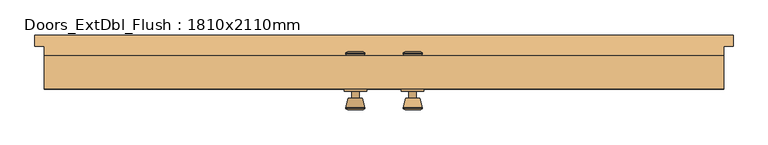
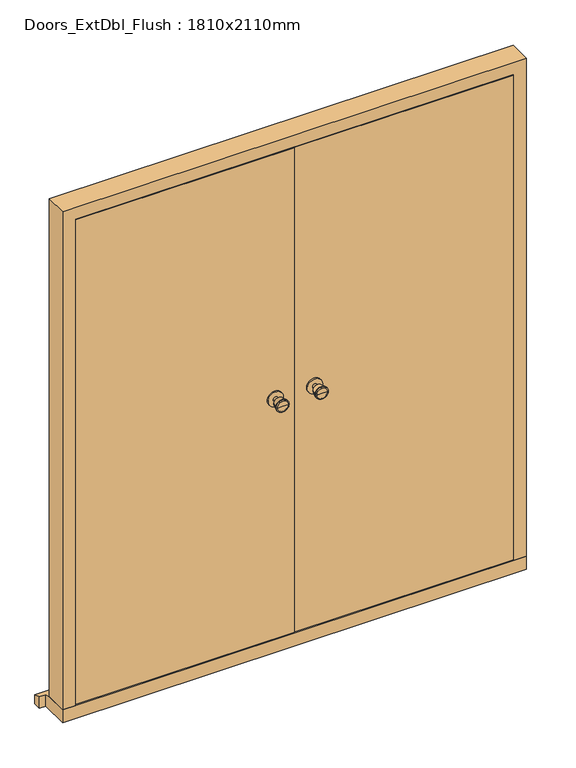
"""IFC4 building model written with IfcOpenShell, lengths in millimetres: door geometry, Doors_ExtDbl_Flush : 1810x2110mm."""

from ifc_helpers import new_model, si_unit, point, frame, frame_2d, origin, place, context, project, spatial, polyline, circle_curve, trimmed, segment, composite_curve, outline, extrude, faceted_brep, source, transform, mapped, element, save
from ifc_brep_helpers import plane_surface, cylinder_surface, revolved_surface, advanced_brep


def doors_extdbl_flush_1810x2110mm_d2e4629e(model_context):
    return source(origin(), model_context, "Body", "SolidModel", [
        advanced_brep(
        [(-76.5, -62.5, 1050.0), (-66.5, -62.5, 1050.0), (-86.5, -62.5, 1050.0), (-96.9758676, -111.5, 1050.0), (-56.0241324, -111.5, 1050.0), (-76.5, -111.5, 1050.0), (-101.5, -109.6721319, 1050.0), (-51.5, -109.6721319, 1050.0), (-101.5, -106.2084537, 1050.0), (-51.5, -106.2084537, 1050.0), (-95.136236, -81.5, 1050.0), (-57.863764, -81.5, 1050.0), (-86.5, -81.5, 1050.0), (-66.5, -81.5, 1050.0)],
        [
            (0, 1),
            (1, 2, circle_curve(frame((-76.5, -62.5, 1050.0), z_axis=(0.0, 1.0, 0.0), x_axis=(1.0, 0.0, 0.0)), 10.0)),
            (2, 0),
            (2, 1, circle_curve(frame((-76.5, -62.5, 1050.0), z_axis=(0.0, 1.0, 0.0), x_axis=(1.0, 0.0, 0.0)), 10.0)),
            (3, 4, circle_curve(frame((-76.5, -111.5, 1050.0), z_axis=(0.0, -1.0, 0.0), x_axis=(1.0, 0.0, 0.0)), 20.4758676)),
            (4, 5),
            (5, 3),
            (4, 3, circle_curve(frame((-76.5, -111.5, 1050.0), z_axis=(0.0, -1.0, 0.0), x_axis=(1.0, 0.0, 0.0)), 20.4758676)),
            (6, 7, circle_curve(frame((-76.5, -109.6721319, 1050.0), z_axis=(0.0, -1.0, 0.0), x_axis=(1.0, 0.0, 0.0)), 25.0)),
            (7, 4),
            (3, 6),
            (7, 6, circle_curve(frame((-76.5, -109.6721319, 1050.0), z_axis=(0.0, -1.0, 0.0), x_axis=(1.0, 0.0, 0.0)), 25.0)),
            (8, 9, circle_curve(frame((-76.5, -106.2084537, 1050.0), z_axis=(0.0, -1.0, 0.0), x_axis=(1.0, 0.0, 0.0)), 25.0)),
            (9, 7),
            (6, 8),
            (9, 8, circle_curve(frame((-76.5, -106.2084537, 1050.0), z_axis=(0.0, -1.0, 0.0), x_axis=(1.0, 0.0, 0.0)), 25.0)),
            (10, 11, circle_curve(frame((-76.5, -81.5, 1050.0), z_axis=(0.0, -1.0, 0.0), x_axis=(1.0, 0.0, 0.0)), 18.636236)),
            (11, 9),
            (8, 10),
            (11, 10, circle_curve(frame((-76.5, -81.5, 1050.0), z_axis=(0.0, -1.0, 0.0), x_axis=(1.0, 0.0, 0.0)), 18.636236)),
            (12, 13, circle_curve(frame((-76.5, -81.5, 1050.0), z_axis=(0.0, -1.0, 0.0), x_axis=(1.0, 0.0, 0.0)), 10.0)),
            (13, 11),
            (10, 12),
            (13, 12, circle_curve(frame((-76.5, -81.5, 1050.0), z_axis=(0.0, -1.0, 0.0), x_axis=(1.0, 0.0, 0.0)), 10.0)),
            (1, 13),
            (12, 2),
        ],
        [
            plane_surface(frame((-76.5, -62.5, 1050.0), z_axis=(0.0, 1.0, 0.0), x_axis=(1.0, 0.0, 0.0))),
            plane_surface(frame((-76.5, -111.5, 1050.0), z_axis=(0.0, -1.0, 0.0), x_axis=(1.0, 0.0, 0.0))),
            revolved_surface(polyline([(-56.0241324, -111.5, 1050.0), (-51.5, -109.6721319, 1050.0)]), (-76.5, -62.5, 1050.0), (0.0, 1.0, 0.0)),
            cylinder_surface(frame((-76.5, -62.5, 1050.0), z_axis=(0.0, 1.0, 0.0), x_axis=(1.0, 0.0, 0.0)), 25.0),
            revolved_surface(polyline([(-51.5, -106.2084537, 1050.0), (-57.863764, -81.5, 1050.0)]), (-76.5, -62.5, 1050.0), (0.0, 1.0, 0.0)),
            plane_surface(frame((-76.5, -81.5, 1050.0), z_axis=(0.0, 1.0, 0.0), x_axis=(1.0, 0.0, 0.0))),
            cylinder_surface(frame((-76.5, -62.5, 1050.0), z_axis=(0.0, 1.0, 0.0), x_axis=(1.0, 0.0, 0.0)), 10.0),
        ],
        [
            (0, [[1, 2, 3]]),
            (0, [[-3, 4, -1]]),
            (1, [[5, 6, 7]]),
            (1, [[8, -7, -6]]),
            (2, [[9, 10, -5, 11]]),
            (2, [[12, -11, -8, -10]]),
            (3, [[13, 14, -9, 15]]),
            (3, [[16, -15, -12, -14]]),
            (4, [[17, 18, -13, 19]]),
            (4, [[20, -19, -16, -18]]),
            (5, [[21, 22, -17, 23]]),
            (5, [[24, -23, -20, -22]]),
            (6, [[-2, 25, -21, 26]]),
            (6, [[-4, -26, -24, -25]]),
        ],
    ),
        extrude(outline(composite_curve([segment(trimmed(circle_curve(frame_2d((1050.0, -76.5)), 30.0), [point((1050.0, -46.5))], [point((1050.0, -106.5))], False, "CARTESIAN"), True, "CONTINUOUS"), segment(trimmed(circle_curve(frame_2d((1050.0, -76.5)), 30.0), [point((1050.0, -106.5))], [point((1050.0, -46.5))], False, "CARTESIAN"), True, "CONTINUOUS")], self_intersect=False)), frame((0.0, -62.5, 0.0), z_axis=(0.0, 1.0, 0.0), x_axis=(0.0, 0.0, 1.0)), (0.0, 0.0, 1.0), 6.0),
        advanced_brep(
        [(-76.5, -6.5, 1050.0), (-86.5, -6.5, 1050.0), (-66.5, -6.5, 1050.0), (-96.9758676, 42.5, 1050.0), (-76.5, 42.5, 1050.0), (-56.0241324, 42.5, 1050.0), (-101.5, 40.6721319, 1050.0), (-51.5, 40.6721319, 1050.0), (-101.5, 37.2084537, 1050.0), (-51.5, 37.2084537, 1050.0), (-95.136236, 12.5, 1050.0), (-57.863764, 12.5, 1050.0), (-86.5, 12.5, 1050.0), (-66.5, 12.5, 1050.0)],
        [
            (0, 1),
            (1, 2, circle_curve(frame((-76.5, -6.5, 1050.0), z_axis=(0.0, -1.0, 0.0), x_axis=(1.0, 0.0, 0.0)), 10.0)),
            (2, 0),
            (2, 1, circle_curve(frame((-76.5, -6.5, 1050.0), z_axis=(0.0, -1.0, 0.0), x_axis=(1.0, 0.0, 0.0)), 10.0)),
            (3, 4),
            (4, 5),
            (5, 3, circle_curve(frame((-76.5, 42.5, 1050.0), z_axis=(0.0, 1.0, 0.0), x_axis=(1.0, 0.0, 0.0)), 20.4758676)),
            (3, 5, circle_curve(frame((-76.5, 42.5, 1050.0), z_axis=(0.0, 1.0, 0.0), x_axis=(1.0, 0.0, 0.0)), 20.4758676)),
            (6, 3),
            (5, 7),
            (7, 6, circle_curve(frame((-76.5, 40.6721319, 1050.0), z_axis=(0.0, 1.0, 0.0), x_axis=(1.0, 0.0, 0.0)), 25.0)),
            (6, 7, circle_curve(frame((-76.5, 40.6721319, 1050.0), z_axis=(0.0, 1.0, 0.0), x_axis=(1.0, 0.0, 0.0)), 25.0)),
            (8, 6),
            (7, 9),
            (9, 8, circle_curve(frame((-76.5, 37.2084537, 1050.0), z_axis=(0.0, 1.0, 0.0), x_axis=(1.0, 0.0, 0.0)), 25.0)),
            (8, 9, circle_curve(frame((-76.5, 37.2084537, 1050.0), z_axis=(0.0, 1.0, 0.0), x_axis=(1.0, 0.0, 0.0)), 25.0)),
            (10, 8),
            (9, 11),
            (11, 10, circle_curve(frame((-76.5, 12.5, 1050.0), z_axis=(0.0, 1.0, 0.0), x_axis=(1.0, 0.0, 0.0)), 18.636236)),
            (10, 11, circle_curve(frame((-76.5, 12.5, 1050.0), z_axis=(0.0, 1.0, 0.0), x_axis=(1.0, 0.0, 0.0)), 18.636236)),
            (12, 10),
            (11, 13),
            (13, 12, circle_curve(frame((-76.5, 12.5, 1050.0), z_axis=(0.0, 1.0, 0.0), x_axis=(1.0, 0.0, 0.0)), 10.0)),
            (12, 13, circle_curve(frame((-76.5, 12.5, 1050.0), z_axis=(0.0, 1.0, 0.0), x_axis=(1.0, 0.0, 0.0)), 10.0)),
            (1, 12),
            (13, 2),
        ],
        [
            plane_surface(frame((-76.5, -6.5, 1050.0), z_axis=(0.0, -1.0, 0.0), x_axis=(1.0, 0.0, 0.0))),
            plane_surface(frame((-76.5, 42.5, 1050.0), z_axis=(0.0, 1.0, 0.0), x_axis=(1.0, 0.0, 0.0))),
            revolved_surface(polyline([(-56.0241324, 42.5, 1050.0), (-51.5, 40.6721319, 1050.0)]), (-76.5, -6.5, 1050.0), (0.0, -1.0, 0.0)),
            cylinder_surface(frame((-76.5, -6.5, 1050.0), z_axis=(0.0, -1.0, 0.0), x_axis=(1.0, 0.0, 0.0)), 25.0),
            revolved_surface(polyline([(-51.5, 37.2084537, 1050.0), (-57.863764, 12.5, 1050.0)]), (-76.5, -6.5, 1050.0), (0.0, -1.0, 0.0)),
            plane_surface(frame((-76.5, 12.5, 1050.0), z_axis=(0.0, -1.0, 0.0), x_axis=(1.0, 0.0, 0.0))),
            cylinder_surface(frame((-76.5, -6.5, 1050.0), z_axis=(0.0, -1.0, 0.0), x_axis=(1.0, 0.0, 0.0)), 10.0),
        ],
        [
            (0, [[1, 2, 3]]),
            (0, [[-3, 4, -1]]),
            (1, [[5, 6, 7]]),
            (1, [[-6, -5, 8]]),
            (2, [[9, -7, 10, 11]]),
            (2, [[-10, -8, -9, 12]]),
            (3, [[13, -11, 14, 15]]),
            (3, [[-14, -12, -13, 16]]),
            (4, [[17, -15, 18, 19]]),
            (4, [[-18, -16, -17, 20]]),
            (5, [[21, -19, 22, 23]]),
            (5, [[-22, -20, -21, 24]]),
            (6, [[25, -23, 26, -2]]),
            (6, [[-26, -24, -25, -4]]),
        ],
    ),
        extrude(outline(composite_curve([segment(trimmed(circle_curve(frame_2d((1050.0, -76.5)), 30.0), [point((1050.0, -46.5))], [point((1050.0, -106.5))], False, "CARTESIAN"), True, "CONTINUOUS"), segment(trimmed(circle_curve(frame_2d((1050.0, -76.5)), 30.0), [point((1050.0, -106.5))], [point((1050.0, -46.5))], False, "CARTESIAN"), True, "CONTINUOUS")], self_intersect=False)), frame((0.0, -12.5, 0.0), z_axis=(0.0, 1.0, 0.0), x_axis=(0.0, 0.0, 1.0)), (0.0, 0.0, 1.0), 6.0),
        advanced_brep(
        [(76.5, -62.5, 1050.0), (86.5, -62.5, 1050.0), (66.5, -62.5, 1050.0), (96.9758676, -111.5, 1050.0), (76.5, -111.5, 1050.0), (56.0241324, -111.5, 1050.0), (101.5, -109.6721319, 1050.0), (51.5, -109.6721319, 1050.0), (101.5, -106.2084537, 1050.0), (51.5, -106.2084537, 1050.0), (95.136236, -81.5, 1050.0), (57.863764, -81.5, 1050.0), (86.5, -81.5, 1050.0), (66.5, -81.5, 1050.0)],
        [
            (0, 1),
            (1, 2, circle_curve(frame((76.5, -62.5, 1050.0), z_axis=(0.0, 1.0, 0.0), x_axis=(-1.0, 0.0, 0.0)), 10.0)),
            (2, 0),
            (2, 1, circle_curve(frame((76.5, -62.5, 1050.0), z_axis=(0.0, 1.0, 0.0), x_axis=(-1.0, 0.0, 0.0)), 10.0)),
            (3, 4),
            (4, 5),
            (5, 3, circle_curve(frame((76.5, -111.5, 1050.0), z_axis=(0.0, -1.0, 0.0), x_axis=(-1.0, 0.0, 0.0)), 20.4758676)),
            (3, 5, circle_curve(frame((76.5, -111.5, 1050.0), z_axis=(0.0, -1.0, 0.0), x_axis=(-1.0, 0.0, 0.0)), 20.4758676)),
            (6, 3),
            (5, 7),
            (7, 6, circle_curve(frame((76.5, -109.6721319, 1050.0), z_axis=(0.0, -1.0, 0.0), x_axis=(-1.0, 0.0, 0.0)), 25.0)),
            (6, 7, circle_curve(frame((76.5, -109.6721319, 1050.0), z_axis=(0.0, -1.0, 0.0), x_axis=(-1.0, 0.0, 0.0)), 25.0)),
            (8, 6),
            (7, 9),
            (9, 8, circle_curve(frame((76.5, -106.2084537, 1050.0), z_axis=(0.0, -1.0, 0.0), x_axis=(-1.0, 0.0, 0.0)), 25.0)),
            (8, 9, circle_curve(frame((76.5, -106.2084537, 1050.0), z_axis=(0.0, -1.0, 0.0), x_axis=(-1.0, 0.0, 0.0)), 25.0)),
            (10, 8),
            (9, 11),
            (11, 10, circle_curve(frame((76.5, -81.5, 1050.0), z_axis=(0.0, -1.0, 0.0), x_axis=(-1.0, 0.0, 0.0)), 18.636236)),
            (10, 11, circle_curve(frame((76.5, -81.5, 1050.0), z_axis=(0.0, -1.0, 0.0), x_axis=(-1.0, 0.0, 0.0)), 18.636236)),
            (12, 10),
            (11, 13),
            (13, 12, circle_curve(frame((76.5, -81.5, 1050.0), z_axis=(0.0, -1.0, 0.0), x_axis=(-1.0, 0.0, 0.0)), 10.0)),
            (12, 13, circle_curve(frame((76.5, -81.5, 1050.0), z_axis=(0.0, -1.0, 0.0), x_axis=(-1.0, 0.0, 0.0)), 10.0)),
            (1, 12),
            (13, 2),
        ],
        [
            plane_surface(frame((76.5, -62.5, 1050.0), z_axis=(0.0, 1.0, 0.0), x_axis=(-1.0, 0.0, 0.0))),
            plane_surface(frame((76.5, -111.5, 1050.0), z_axis=(0.0, -1.0, 0.0), x_axis=(-1.0, 0.0, 0.0))),
            revolved_surface(polyline([(56.0241324, -111.5, 1050.0), (51.5, -109.6721319, 1050.0)]), (76.5, -62.5, 1050.0), (0.0, 1.0, 0.0)),
            cylinder_surface(frame((76.5, -62.5, 1050.0), z_axis=(0.0, 1.0, 0.0), x_axis=(-1.0, 0.0, 0.0)), 25.0),
            revolved_surface(polyline([(51.5, -106.2084537, 1050.0), (57.863764, -81.5, 1050.0)]), (76.5, -62.5, 1050.0), (0.0, 1.0, 0.0)),
            plane_surface(frame((76.5, -81.5, 1050.0), z_axis=(0.0, 1.0, 0.0), x_axis=(-1.0, 0.0, 0.0))),
            cylinder_surface(frame((76.5, -62.5, 1050.0), z_axis=(0.0, 1.0, 0.0), x_axis=(-1.0, 0.0, 0.0)), 10.0),
        ],
        [
            (0, [[1, 2, 3]]),
            (0, [[-3, 4, -1]]),
            (1, [[5, 6, 7]]),
            (1, [[-6, -5, 8]]),
            (2, [[9, -7, 10, 11]]),
            (2, [[-10, -8, -9, 12]]),
            (3, [[13, -11, 14, 15]]),
            (3, [[-14, -12, -13, 16]]),
            (4, [[17, -15, 18, 19]]),
            (4, [[-18, -16, -17, 20]]),
            (5, [[21, -19, 22, 23]]),
            (5, [[-22, -20, -21, 24]]),
            (6, [[25, -23, 26, -2]]),
            (6, [[-26, -24, -25, -4]]),
        ],
    ),
        extrude(outline(composite_curve([segment(trimmed(circle_curve(frame_2d((1050.0, 76.5)), 30.0), [point((1050.0, 46.5))], [point((1050.0, 106.5))], False, "CARTESIAN"), True, "CONTINUOUS"), segment(trimmed(circle_curve(frame_2d((1050.0, 76.5)), 30.0), [point((1050.0, 106.5))], [point((1050.0, 46.5))], False, "CARTESIAN"), True, "CONTINUOUS")], self_intersect=False)), frame((0.0, -62.5, 0.0), z_axis=(0.0, 1.0, 0.0), x_axis=(0.0, 0.0, 1.0)), (0.0, 0.0, 1.0), 6.0),
        advanced_brep(
        [(76.5, -6.5, 1050.0), (66.5, -6.5, 1050.0), (86.5, -6.5, 1050.0), (96.9758676, 42.5, 1050.0), (56.0241324, 42.5, 1050.0), (76.5, 42.5, 1050.0), (101.5, 40.6721319, 1050.0), (51.5, 40.6721319, 1050.0), (101.5, 37.2084537, 1050.0), (51.5, 37.2084537, 1050.0), (95.136236, 12.5, 1050.0), (57.863764, 12.5, 1050.0), (86.5, 12.5, 1050.0), (66.5, 12.5, 1050.0)],
        [
            (0, 1),
            (1, 2, circle_curve(frame((76.5, -6.5, 1050.0), z_axis=(0.0, -1.0, 0.0), x_axis=(-1.0, 0.0, 0.0)), 10.0)),
            (2, 0),
            (2, 1, circle_curve(frame((76.5, -6.5, 1050.0), z_axis=(0.0, -1.0, 0.0), x_axis=(-1.0, 0.0, 0.0)), 10.0)),
            (3, 4, circle_curve(frame((76.5, 42.5, 1050.0), z_axis=(0.0, 1.0, 0.0), x_axis=(-1.0, 0.0, 0.0)), 20.4758676)),
            (4, 5),
            (5, 3),
            (4, 3, circle_curve(frame((76.5, 42.5, 1050.0), z_axis=(0.0, 1.0, 0.0), x_axis=(-1.0, 0.0, 0.0)), 20.4758676)),
            (6, 7, circle_curve(frame((76.5, 40.6721319, 1050.0), z_axis=(0.0, 1.0, 0.0), x_axis=(-1.0, 0.0, 0.0)), 25.0)),
            (7, 4),
            (3, 6),
            (7, 6, circle_curve(frame((76.5, 40.6721319, 1050.0), z_axis=(0.0, 1.0, 0.0), x_axis=(-1.0, 0.0, 0.0)), 25.0)),
            (8, 9, circle_curve(frame((76.5, 37.2084537, 1050.0), z_axis=(0.0, 1.0, 0.0), x_axis=(-1.0, 0.0, 0.0)), 25.0)),
            (9, 7),
            (6, 8),
            (9, 8, circle_curve(frame((76.5, 37.2084537, 1050.0), z_axis=(0.0, 1.0, 0.0), x_axis=(-1.0, 0.0, 0.0)), 25.0)),
            (10, 11, circle_curve(frame((76.5, 12.5, 1050.0), z_axis=(0.0, 1.0, 0.0), x_axis=(-1.0, 0.0, 0.0)), 18.636236)),
            (11, 9),
            (8, 10),
            (11, 10, circle_curve(frame((76.5, 12.5, 1050.0), z_axis=(0.0, 1.0, 0.0), x_axis=(-1.0, 0.0, 0.0)), 18.636236)),
            (12, 13, circle_curve(frame((76.5, 12.5, 1050.0), z_axis=(0.0, 1.0, 0.0), x_axis=(-1.0, 0.0, 0.0)), 10.0)),
            (13, 11),
            (10, 12),
            (13, 12, circle_curve(frame((76.5, 12.5, 1050.0), z_axis=(0.0, 1.0, 0.0), x_axis=(-1.0, 0.0, 0.0)), 10.0)),
            (1, 13),
            (12, 2),
        ],
        [
            plane_surface(frame((76.5, -6.5, 1050.0), z_axis=(0.0, -1.0, 0.0), x_axis=(-1.0, 0.0, 0.0))),
            plane_surface(frame((76.5, 42.5, 1050.0), z_axis=(0.0, 1.0, 0.0), x_axis=(-1.0, 0.0, 0.0))),
            revolved_surface(polyline([(56.0241324, 42.5, 1050.0), (51.5, 40.6721319, 1050.0)]), (76.5, -6.5, 1050.0), (0.0, -1.0, 0.0)),
            cylinder_surface(frame((76.5, -6.5, 1050.0), z_axis=(0.0, -1.0, 0.0), x_axis=(-1.0, 0.0, 0.0)), 25.0),
            revolved_surface(polyline([(51.5, 37.2084537, 1050.0), (57.863764, 12.5, 1050.0)]), (76.5, -6.5, 1050.0), (0.0, -1.0, 0.0)),
            plane_surface(frame((76.5, 12.5, 1050.0), z_axis=(0.0, -1.0, 0.0), x_axis=(-1.0, 0.0, 0.0))),
            cylinder_surface(frame((76.5, -6.5, 1050.0), z_axis=(0.0, -1.0, 0.0), x_axis=(-1.0, 0.0, 0.0)), 10.0),
        ],
        [
            (0, [[1, 2, 3]]),
            (0, [[-3, 4, -1]]),
            (1, [[5, 6, 7]]),
            (1, [[8, -7, -6]]),
            (2, [[9, 10, -5, 11]]),
            (2, [[12, -11, -8, -10]]),
            (3, [[13, 14, -9, 15]]),
            (3, [[16, -15, -12, -14]]),
            (4, [[17, 18, -13, 19]]),
            (4, [[20, -19, -16, -18]]),
            (5, [[21, 22, -17, 23]]),
            (5, [[24, -23, -20, -22]]),
            (6, [[-2, 25, -21, 26]]),
            (6, [[-4, -26, -24, -25]]),
        ],
    ),
        extrude(outline(composite_curve([segment(trimmed(circle_curve(frame_2d((1050.0, 76.5)), 30.0), [point((1050.0, 46.5))], [point((1050.0, 106.5))], False, "CARTESIAN"), True, "CONTINUOUS"), segment(trimmed(circle_curve(frame_2d((1050.0, 76.5)), 30.0), [point((1050.0, 106.5))], [point((1050.0, 46.5))], False, "CARTESIAN"), True, "CONTINUOUS")], self_intersect=False)), frame((0.0, -12.5, 0.0), z_axis=(0.0, 1.0, 0.0), x_axis=(0.0, 0.0, 1.0)), (0.0, 0.0, 1.0), 6.0),
        faceted_brep([(834.5, 32.5, 54.5), (905.0, 32.5, 54.5), (905.0, -56.5, 54.5), (856.5, -56.5, 54.5), (856.5, -9.5, 54.5), (834.5, -9.5, 54.5), (834.5, 32.5, 2039.5), (-834.5, 32.5, 2039.5), (-834.5, 32.5, 54.5), (-905.0, 32.5, 54.5), (-905.0, 32.5, 2110.0), (905.0, 32.5, 2110.0), (905.0, -56.5, 2110.0), (-905.0, -56.5, 2110.0), (-905.0, -56.5, 54.5), (-856.5, -56.5, 54.5), (-856.5, -56.5, 2061.5), (856.5, -56.5, 2061.5), (856.5, -9.5, 2061.5), (-856.5, -9.5, 2061.5), (-856.5, -9.5, 54.5), (-834.5, -9.5, 54.5), (-834.5, -9.5, 2039.5), (834.5, -9.5, 2039.5)], [[[0, 1, 2, 3, 4, 5]], [[1, 0, 6, 7, 8, 9, 10, 11]], [[2, 1, 11, 12]], [[3, 2, 12, 13, 14, 15, 16, 17]], [[4, 3, 17, 18]], [[5, 4, 18, 19, 20, 21, 22, 23]], [[0, 5, 23, 6]], [[12, 11, 10, 13]], [[18, 17, 16, 19]], [[6, 23, 22, 7]], [[8, 21, 20, 15, 14, 9]], [[13, 10, 9, 14]], [[19, 16, 15, 20]], [[7, 22, 21, 8]]]),
        faceted_brep([(930.0, 87.5, 0.0), (930.0, 87.5, 38.5947221), (930.0, 57.5, 47.2703282), (930.0, 57.5, 0.0), (-930.0, 87.5, 38.5947221), (-930.0, 87.5, 0.0), (-930.0, 57.5, 0.0), (-930.0, 57.5, 47.2703282), (905.0, 57.5, 0.0), (905.0, -56.5, 0.0), (-905.0, -56.5, 0.0), (-905.0, 57.5, 0.0), (-905.0, 57.5, 47.2703282), (-905.0, 32.5, 54.5), (905.0, 32.5, 54.5), (905.0, 57.5, 47.2703282), (-905.0, -56.5, 54.5), (905.0, -56.5, 54.5)], [[[0, 1, 2, 3]], [[4, 5, 6, 7]], [[5, 0, 3, 8, 9, 10, 11, 6]], [[1, 0, 5, 4]], [[1, 4, 7, 12, 13, 14, 15, 2]], [[13, 16, 17, 14]], [[16, 10, 9, 17]], [[12, 11, 10, 16, 13]], [[11, 12, 7, 6]], [[8, 15, 14, 17, 9]], [[15, 8, 3, 2]]]),
        extrude(outline(polyline([(853.5, -56.5), (1.5, -56.5), (1.5, -12.5), (853.5, -12.5), (853.5, -56.5)])), frame((0.0, 0.0, 58.5), z_axis=(0.0, 0.0, 1.0), x_axis=(1.0, 0.0, 0.0)), (0.0, 0.0, 1.0), 2000.0),
        extrude(outline(polyline([(-1.5, -56.5), (-853.5, -56.5), (-853.5, -12.5), (-1.5, -12.5), (-1.5, -56.5)])), frame((0.0, 0.0, 58.5), z_axis=(0.0, 0.0, 1.0), x_axis=(1.0, 0.0, 0.0)), (0.0, 0.0, 1.0), 2000.0),
    ])


if __name__ == "__main__":
    model = new_model("IFC4")
    model_context = context("Model", 3, world=origin())
    ifc_project = project(units=[si_unit("LENGTHUNIT", "METRE", prefix="MILLI")], contexts=[model_context])
    site = spatial("IfcSite", under=ifc_project)
    building = spatial("IfcBuilding", under=site)
    placement = place(None, origin())
    doors_extdbl_flush_1810x2110mm_shape = doors_extdbl_flush_1810x2110mm_d2e4629e(model_context)
    element("IfcDoor", 1, ObjectType="Doors_ExtDbl_Flush : 1810x2110mm", at=placement, inside=building, context=model_context, shape_type="MappedRepresentation", body=[
        mapped(doors_extdbl_flush_1810x2110mm_shape, transform((0.0, 0.0, 0.0), x_axis=(1.0, 0.0, 0.0), y_axis=(0.0, 1.0, 0.0), z_axis=(0.0, 0.0, 1.0))),
    ])
    save(model, "model.ifc")

# Revit data of these elements
# Type "Doors_ExtDbl_Flush : 1810x2110mm"
#   Type Mark = "44"
#   Type Comments = "External Double"
#   Operation = "DoubleDoorSingleSwing"
#   Keynote = "L20"
#   Analytic Construction = "Metal"
#   Wrap Layers (Ext) from Ext = 102.5 mm
#   Wrap Layers (Int) from Ext = 177.5 mm
#   Thickness = 44 mm
#   Rough Width = 1810 mm
#   Rough Height = 2110 mm
#   O/A Frame Width = 64 mm
#   Heat Transfer Coefficient (U) = 3.7021 W/(m²·K)
#   Handle Z Distance = 1050 mm
#   FrameWidth = 42 mm
#   FrameOffset - External = 25 mm
#   FrameDepth = 89 mm
#   Door Panel Width = 852 mm
#   Door Panel Thickness = 44 mm
#   Door Panel Height = 2000 mm
#   Cill Thickness = 54.5 mm
#   Cill Projection = 30 mm
#   Handle X Distance = 75 mm
#   Height = 2110 mm
#   Structural Tolerance = 6.5 mm
#   Tolerance = 3 mm
#   Undercut = 4 mm
#   Width = 1810 mm
#   Cill Extension = 25 mm
#   Cavity Closer Width = 50 mm
#   Cavity Closer Offset from Ext = 102.5 mm
#   Cavity Closer Depth = 85 mm
#   Define Thermal Properties by = 0
#   Vis - Ironmongery = yes
#   Vis - Cavity Closers = yes
#   Function = 1
#   Material Door = Door - Panel
#   Material Frame = Door - Frame/Mullion
#   Material Ironmongery = Door - Handle
#   Visual Light Transmittance = 0
#   Thermal Resistance (R) = 0
#   Solar Heat Gain Coefficient = 0
#   Wall Closure = (empty or 0)
# Element 1 (IfcDoor, "Doors_ExtDbl_Flush : 1810x2110mm")
#   Materials on its faces: "Door - Handle", "Door - Frame/Mullion", "Door - Panel"
# Materials
#   "Door - Panel": class "Wood", colour RGB 210 159 95, transparency 0, Keynote = "L20", Cost = 0
#   "Door - Frame/Mullion": class "Wood", colour RGB 212 179 113, transparency 0, Keynote = "L20", Cost = 0
#   "Door - Handle": class "Miscellaneous", colour RGB 0 0 0, transparency 0, Keynote = "P21", Cost = 0
